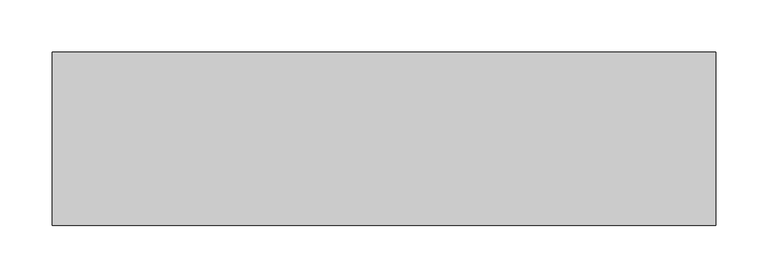
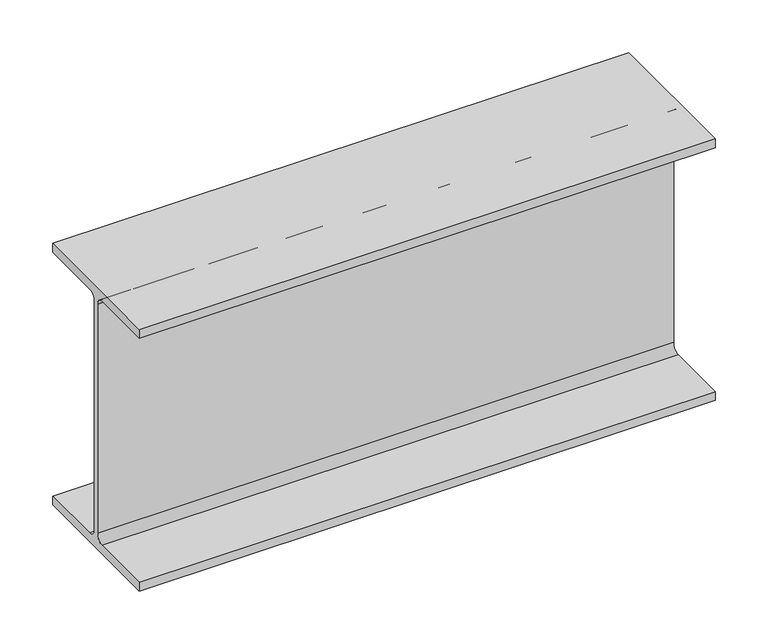
"""IFC4 building model written with IfcOpenShell, lengths in millimetres: beam geometry, Steel Beam_H-KSD3502 : H_SB_ASB_H-300x150x6.5x9."""

import ifcopenshell
import ifcopenshell.guid

model = None  # the IFC model being written
_history = None  # IfcOwnerHistory: only IFC2X3 demands one
_inside = {}  # id of a spatial element -> (the spatial element, [elements in it])
_under = {}  # id of a project, library or spatial element -> (it, [spatial elements below it])
_declared = {}  # id of a project -> (the project, [libraries it declares])
_typed = {}  # id of a type object -> (the type object, [elements of that type])
_made_of = {}  # id of a material, layer set ... -> (it, [elements and type objects made of it])


def new_model(schema):
    """Start an empty IFC model of exactly this schema.

    Asked for "IFC4X3", IfcOpenShell would pick the latest addendum, in which some entities
    have other attributes; the version numbers below select the first issue.
    IFC2X3 requires an IfcOwnerHistory on every rooted entity: one is made here for all.
    """
    global model, _history
    if schema == "IFC4X3":
        model = ifcopenshell.file(schema_version=(4, 3, 0, 0))
    else:
        model = ifcopenshell.file(schema=schema)
    _inside.clear()
    _under.clear()
    _declared.clear()
    _typed.clear()
    _made_of.clear()
    _history = None
    if model.schema == "IFC2X3":
        org = make("IfcOrganization", Name="unknown")
        user = make(
            "IfcPersonAndOrganization",
            ThePerson=make("IfcPerson", FamilyName="unknown"),
            TheOrganization=org,
        )
        app = make(
            "IfcApplication",
            ApplicationDeveloper=org,
            Version="unknown",
            ApplicationFullName="unknown",
            ApplicationIdentifier="unknown",
        )
        _history = make(
            "IfcOwnerHistory",
            OwningUser=user,
            OwningApplication=app,
            ChangeAction="ADDED",
            CreationDate=0,
        )
    return model


def make(cls, **values):
    """One entity of the class cls with the attributes given. An attribute that is None is left unset."""
    return model.create_entity(
        cls, **{name: value for name, value in values.items() if value is not None}
    )


def rooted(cls, **values):
    """An entity with a GlobalId (a new one), such as an element, a storey or a relation."""
    return make(cls, GlobalId=ifcopenshell.guid.new(), OwnerHistory=_history, **values)


def si_unit(unit_type, name, prefix=None):
    """IfcSIUnit, for example si_unit("LENGTHUNIT", "METRE", prefix="MILLI")."""
    return make("IfcSIUnit", UnitType=unit_type, Prefix=prefix, Name=name)


def assignment(units):
    """IfcUnitAssignment: the units of a project."""
    return None if units is None else make("IfcUnitAssignment", Units=units)


def point(xyz):
    """IfcCartesianPoint."""
    return None if xyz is None else make("IfcCartesianPoint", Coordinates=xyz)


def direction(xyz):
    """IfcDirection."""
    return None if xyz is None else make("IfcDirection", DirectionRatios=xyz)


def frame(location, z_axis=None, x_axis=None):
    """IfcAxis2Placement3D, a coordinate frame: its origin and axes. An axis left out is left unset."""
    return make(
        "IfcAxis2Placement3D",
        Location=point(location),
        Axis=direction(z_axis),
        RefDirection=direction(x_axis),
    )


def frame_2d(location, x_axis=None):
    """IfcAxis2Placement2D, a coordinate frame in the plane: its origin and x axis."""
    return make(
        "IfcAxis2Placement2D", Location=point(location), RefDirection=direction(x_axis)
    )


def origin():
    """The frame at (0, 0, 0) with its axes left unset."""
    return frame((0.0, 0.0, 0.0))


def place(relative_to, where):
    """IfcLocalPlacement: puts the frame where relative to a parent placement (None: the world)."""
    return make(
        "IfcLocalPlacement", PlacementRelTo=relative_to, RelativePlacement=where
    )


def context(
    kind, dimensions, precision=None, world=None, true_north=None, identifier=None
):
    """IfcGeometricRepresentationContext, for example the 3D "Model" context."""
    return make(
        "IfcGeometricRepresentationContext",
        ContextIdentifier=identifier,
        ContextType=kind,
        CoordinateSpaceDimension=dimensions,
        Precision=precision,
        WorldCoordinateSystem=world,
        TrueNorth=true_north,
    )


def project(units=None, contexts=None):
    """IfcProject with its units and contexts."""
    return rooted(
        "IfcProject",
        Name="project",
        RepresentationContexts=contexts,
        UnitsInContext=assignment(units),
    )


def spatial(cls, under=None, at=None, **own):
    """A site, building, storey or space (cls), placed at a placement, below another one or the project."""
    s = rooted(cls, ObjectPlacement=at, **own)
    if under is not None:
        _under.setdefault(under.id(), (under, []))[1].append(s)
    return s


def polyline(points):
    """IfcPolyline through the points."""
    return make("IfcPolyline", Points=[point(p) for p in points])


def circle_curve(where, radius):
    """IfcCircle in the frame where."""
    return make("IfcCircle", Position=where, Radius=radius)


def trimmed(basis, trim1, trim2, sense, master):
    """IfcTrimmedCurve: the piece of a basis curve between two trims."""
    return make(
        "IfcTrimmedCurve",
        BasisCurve=basis,
        Trim1=trim1,
        Trim2=trim2,
        SenseAgreement=sense,
        MasterRepresentation=master,
    )


def segment(curve, same_sense, transition):
    """IfcCompositeCurveSegment."""
    return make(
        "IfcCompositeCurveSegment",
        Transition=transition,
        SameSense=same_sense,
        ParentCurve=curve,
    )


def composite_curve(segments, self_intersect=None):
    """IfcCompositeCurve: segments joined end to end."""
    return make("IfcCompositeCurve", Segments=segments, SelfIntersect=self_intersect)


def outline(outer, holes=None, kind="AREA"):
    """IfcArbitraryClosedProfileDef: a profile drawn as a closed curve; with holes, ...WithVoids."""
    if holes is None:
        return make("IfcArbitraryClosedProfileDef", ProfileType=kind, OuterCurve=outer)
    return make(
        "IfcArbitraryProfileDefWithVoids",
        ProfileType=kind,
        OuterCurve=outer,
        InnerCurves=holes,
    )


def extrude(swept, where, along, depth):
    """IfcExtrudedAreaSolid: the profile swept, set in the frame where, extruded along a direction by depth."""
    return make(
        "IfcExtrudedAreaSolid",
        SweptArea=swept,
        Position=where,
        ExtrudedDirection=direction(along),
        Depth=depth,
    )


def shape(context_of_items, identifier, shape_type, items):
    """IfcShapeRepresentation: the items that make up one representation, for example the "Body"."""
    return make(
        "IfcShapeRepresentation",
        ContextOfItems=context_of_items,
        RepresentationIdentifier=identifier,
        RepresentationType=shape_type,
        Items=items,
    )


def source(mapping_origin, context_of_items, identifier, shape_type, items):
    """IfcRepresentationMap: a shape defined once, which mapped items show again and again."""
    return make(
        "IfcRepresentationMap",
        MappingOrigin=mapping_origin,
        MappedRepresentation=shape(context_of_items, identifier, shape_type, items),
    )


def transform(
    local_origin,
    x_axis=None,
    y_axis=None,
    z_axis=None,
    scale=None,
    scale2=None,
    scale3=None,
    uniform=True,
):
    """IfcCartesianTransformationOperator3D, or its non-uniform kind. x_axis, y_axis, z_axis: its Axis1, 2, 3."""
    if uniform:
        return make(
            "IfcCartesianTransformationOperator3D",
            Axis1=direction(x_axis),
            Axis2=direction(y_axis),
            LocalOrigin=point(local_origin),
            Scale=scale,
            Axis3=direction(z_axis),
        )
    return make(
        "IfcCartesianTransformationOperator3DnonUniform",
        Axis1=direction(x_axis),
        Axis2=direction(y_axis),
        LocalOrigin=point(local_origin),
        Scale=scale,
        Axis3=direction(z_axis),
        Scale2=scale2,
        Scale3=scale3,
    )


def mapped(mapping_source, mapping_target):
    """IfcMappedItem: shows the shape of a source again, moved by a transform."""
    return make(
        "IfcMappedItem", MappingSource=mapping_source, MappingTarget=mapping_target
    )


def made_of(thing, what):
    """Note that an element or type object is made of a material, layer set ...; save() writes the relation."""
    if what is not None:
        _made_of.setdefault(what.id(), (what, []))[1].append(thing)
    return thing


def element(
    cls,
    number,
    at=None,
    inside=None,
    cuts=None,
    type_object=None,
    material=None,
    context=None,
    identifier="Body",
    shape_type=None,
    held_by="IfcProductDefinitionShape",
    body=None,
    shapes=None,
    **own,
):
    """One element of the class cls, such as IfcWall. Its Tag is "e" and its number.

    at: its placement. inside: the storey or other place that contains it. cuts: it is an
    opening in that element (IfcRelVoidsElement). A single representation is given by context,
    identifier, shape_type and body (its items); several are given by shapes. held_by: the class
    of the entity that holds the representations. save() writes the other relations.
    """
    e = rooted(cls, Tag="e%d" % number, ObjectPlacement=at, **own)
    if body is not None:
        shapes = [shape(context, identifier, shape_type, body)]
    if shapes is not None:
        e.Representation = make(held_by, Representations=shapes)
    if inside is not None:
        _inside.setdefault(inside.id(), (inside, []))[1].append(e)
    if cuts is not None:
        rooted(
            "IfcRelVoidsElement", RelatingBuildingElement=cuts, RelatedOpeningElement=e
        )
    if type_object is not None:
        _typed.setdefault(type_object.id(), (type_object, []))[1].append(e)
    return made_of(e, material)


def aggregate(whole, parts):
    """IfcRelAggregates: a whole, such as a stair, and the parts it consists of."""
    return rooted("IfcRelAggregates", RelatingObject=whole, RelatedObjects=parts)


def save(model, path):
    """Write the relations noted so far, then the file.

    IfcRelAggregates (storeys below a building ...), IfcRelContainedInSpatialStructure (elements
    in a storey), IfcRelDefinesByType, IfcRelAssociatesMaterial and IfcRelDeclares: one each for
    every whole, place, type object, material and project.
    """
    for whole, parts in _under.values():
        aggregate(whole, parts)
    for where, things in _inside.values():
        rooted(
            "IfcRelContainedInSpatialStructure",
            RelatedElements=things,
            RelatingStructure=where,
        )
    for kind, things in _typed.values():
        rooted("IfcRelDefinesByType", RelatedObjects=things, RelatingType=kind)
    for what, things in _made_of.values():
        rooted("IfcRelAssociatesMaterial", RelatedObjects=things, RelatingMaterial=what)
    for by, libraries in _declared.values():
        rooted("IfcRelDeclares", RelatingContext=by, RelatedDefinitions=libraries)
    model.write(path)


def beam_aa7ca716(model_context):
    return source(origin(), model_context, "Body", "SweptSolid", [
        extrude(outline(composite_curve([segment(polyline([(-82.5, -141.5), (-11.9, -141.5)]), True, "CONTINUOUS"), segment(trimmed(circle_curve(frame_2d((-11.9, -132.6)), 8.9), [point((-11.9, -141.5))], [point((-3.0, -132.6))], True, "CARTESIAN"), True, "CONTINUOUS"), segment(polyline([(-3.0, -132.6), (-3.0, 132.6)]), True, "CONTINUOUS"), segment(trimmed(circle_curve(frame_2d((-11.9, 132.6)), 8.9), [point((-3.0, 132.6))], [point((-11.9, 141.5))], True, "CARTESIAN"), True, "CONTINUOUS"), segment(polyline([(-11.9, 141.5), (-82.5, 141.5), (-82.5, 151.7), (82.5, 151.7), (82.5, 141.5), (11.9, 141.5)]), True, "CONTINUOUS"), segment(trimmed(circle_curve(frame_2d((11.9, 132.6)), 8.9), [point((11.9, 141.5))], [point((3.0, 132.6))], True, "CARTESIAN"), True, "CONTINUOUS"), segment(polyline([(3.0, 132.6), (3.0, -132.6)]), True, "CONTINUOUS"), segment(trimmed(circle_curve(frame_2d((11.9, -132.6)), 8.9), [point((3.0, -132.6))], [point((11.9, -141.5))], True, "CARTESIAN"), True, "CONTINUOUS"), segment(polyline([(11.9, -141.5), (82.5, -141.5), (82.5, -151.7), (-82.5, -151.7), (-82.5, -141.5)]), True, "CONTINUOUS")], self_intersect=False)), frame((-282.3, 0.0, 0.0), z_axis=(1.0, 0.0, 0.0), x_axis=(0.0, 1.0, 0.0)), (0.0, 0.0, 1.0), 632.1),
    ])


if __name__ == "__main__":
    model = new_model("IFC4")
    model_context = context("Model", 3, world=origin())
    ifc_project = project(units=[si_unit("LENGTHUNIT", "METRE", prefix="MILLI")], contexts=[model_context])
    site = spatial("IfcSite", under=ifc_project)
    building = spatial("IfcBuilding", under=site)
    placement = place(None, origin())
    beam_shape = beam_aa7ca716(model_context)
    element("IfcBeam", 1, ObjectType="Steel Beam_H-KSD3502 : H_SB_ASB_H-300x150x6.5x9", at=placement, inside=building, context=model_context, shape_type="MappedRepresentation", body=[
        mapped(beam_shape, transform((0.0, 0.0, 0.0), x_axis=(1.0, 0.0, 0.0), y_axis=(0.0, 1.0, 0.0), z_axis=(0.0, 0.0, 1.0))),
    ])
    save(model, "model.ifc")

# Revit data of these elements
# Type "Steel Beam_H-KSD3502 : H_SB_ASB_H-300x150x6.5x9"
#   Width = 15.0 cm
#   Web Thickness = 0.65 cm
#   Web Fillet = 1.3 cm
#   Warping Constant = 107174.0 cm⁶
#   Torsional Moment of Inertia = 9.9539 cm⁴
#   Torsional Modulus = 1.0 cm³
#   Section Area = 46.78 cm²
#   Plastic Modulus weak axis = 105.0 cm³
#   Plastic Modulus strong axis = 542.0 cm³
#   Perimeter = 1.17 m²/m
#   Nominal Weight = 36.70 kgf/m
#   Moment of Inertia weak axis = 508.00 cm⁴
#   Moment of Inertia strong axis = 7210.00 cm⁴
#   Height = 30.0 cm
#   Flange Thickness = 0.9 cm
#   Elastic Modulus weak axis = 67.7 cm³
#   Elastic Modulus strong axis = 481.0 cm³
#   Centroid Vertical = 15.0 cm
#   Centroid Horizontal = 7.5 cm
#   Length [instance default] = 1.5240 m
#   Structural Material [instance default] = Steel, 45-345
#   Assembly Code = ""
# Element 1 (IfcBeam, "Steel Beam_H-KSD3502 : H_SB_ASB_H-300x150x6.5x9")
#   Structural Material = none
# Materials
#   "Steel, 45-345": class "Metal", colour RGB 189 187 185, transparency 0, Description = "Steel 345 MPa", Cost = 0
